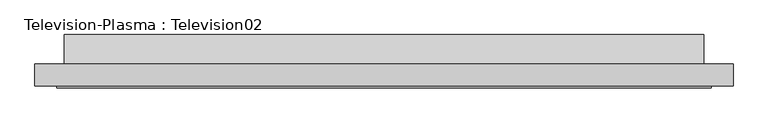
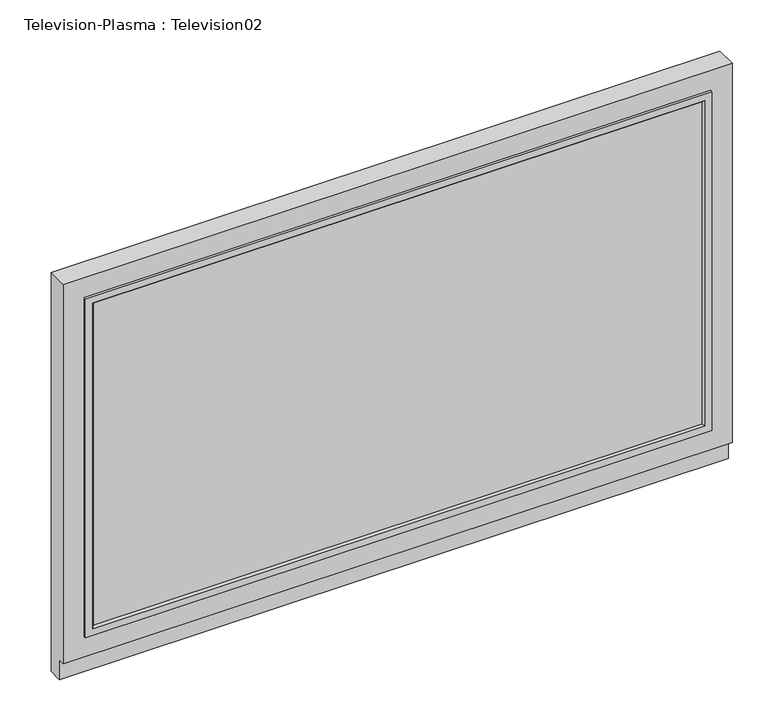
"""IFC4 building model written with IfcOpenShell, lengths in millimetres: furniture geometry, Television-Plasma : Television02."""

import ifcopenshell
import ifcopenshell.guid

model = None  # the IFC model being written
_history = None  # IfcOwnerHistory: only IFC2X3 demands one
_inside = {}  # id of a spatial element -> (the spatial element, [elements in it])
_under = {}  # id of a project, library or spatial element -> (it, [spatial elements below it])
_declared = {}  # id of a project -> (the project, [libraries it declares])
_typed = {}  # id of a type object -> (the type object, [elements of that type])
_made_of = {}  # id of a material, layer set ... -> (it, [elements and type objects made of it])


def new_model(schema):
    """Start an empty IFC model of exactly this schema.

    Asked for "IFC4X3", IfcOpenShell would pick the latest addendum, in which some entities
    have other attributes; the version numbers below select the first issue.
    IFC2X3 requires an IfcOwnerHistory on every rooted entity: one is made here for all.
    """
    global model, _history
    if schema == "IFC4X3":
        model = ifcopenshell.file(schema_version=(4, 3, 0, 0))
    else:
        model = ifcopenshell.file(schema=schema)
    _inside.clear()
    _under.clear()
    _declared.clear()
    _typed.clear()
    _made_of.clear()
    _history = None
    if model.schema == "IFC2X3":
        org = make("IfcOrganization", Name="unknown")
        user = make(
            "IfcPersonAndOrganization",
            ThePerson=make("IfcPerson", FamilyName="unknown"),
            TheOrganization=org,
        )
        app = make(
            "IfcApplication",
            ApplicationDeveloper=org,
            Version="unknown",
            ApplicationFullName="unknown",
            ApplicationIdentifier="unknown",
        )
        _history = make(
            "IfcOwnerHistory",
            OwningUser=user,
            OwningApplication=app,
            ChangeAction="ADDED",
            CreationDate=0,
        )
    return model


def make(cls, **values):
    """One entity of the class cls with the attributes given. An attribute that is None is left unset."""
    return model.create_entity(
        cls, **{name: value for name, value in values.items() if value is not None}
    )


def rooted(cls, **values):
    """An entity with a GlobalId (a new one), such as an element, a storey or a relation."""
    return make(cls, GlobalId=ifcopenshell.guid.new(), OwnerHistory=_history, **values)


def si_unit(unit_type, name, prefix=None):
    """IfcSIUnit, for example si_unit("LENGTHUNIT", "METRE", prefix="MILLI")."""
    return make("IfcSIUnit", UnitType=unit_type, Prefix=prefix, Name=name)


def assignment(units):
    """IfcUnitAssignment: the units of a project."""
    return None if units is None else make("IfcUnitAssignment", Units=units)


def point(xyz):
    """IfcCartesianPoint."""
    return None if xyz is None else make("IfcCartesianPoint", Coordinates=xyz)


def direction(xyz):
    """IfcDirection."""
    return None if xyz is None else make("IfcDirection", DirectionRatios=xyz)


def frame(location, z_axis=None, x_axis=None):
    """IfcAxis2Placement3D, a coordinate frame: its origin and axes. An axis left out is left unset."""
    return make(
        "IfcAxis2Placement3D",
        Location=point(location),
        Axis=direction(z_axis),
        RefDirection=direction(x_axis),
    )


def origin():
    """The frame at (0, 0, 0) with its axes left unset."""
    return frame((0.0, 0.0, 0.0))


def place(relative_to, where):
    """IfcLocalPlacement: puts the frame where relative to a parent placement (None: the world)."""
    return make(
        "IfcLocalPlacement", PlacementRelTo=relative_to, RelativePlacement=where
    )


def context(
    kind, dimensions, precision=None, world=None, true_north=None, identifier=None
):
    """IfcGeometricRepresentationContext, for example the 3D "Model" context."""
    return make(
        "IfcGeometricRepresentationContext",
        ContextIdentifier=identifier,
        ContextType=kind,
        CoordinateSpaceDimension=dimensions,
        Precision=precision,
        WorldCoordinateSystem=world,
        TrueNorth=true_north,
    )


def project(units=None, contexts=None):
    """IfcProject with its units and contexts."""
    return rooted(
        "IfcProject",
        Name="project",
        RepresentationContexts=contexts,
        UnitsInContext=assignment(units),
    )


def spatial(cls, under=None, at=None, **own):
    """A site, building, storey or space (cls), placed at a placement, below another one or the project."""
    s = rooted(cls, ObjectPlacement=at, **own)
    if under is not None:
        _under.setdefault(under.id(), (under, []))[1].append(s)
    return s


def polyline(points):
    """IfcPolyline through the points."""
    return make("IfcPolyline", Points=[point(p) for p in points])


def outline(outer, holes=None, kind="AREA"):
    """IfcArbitraryClosedProfileDef: a profile drawn as a closed curve; with holes, ...WithVoids."""
    if holes is None:
        return make("IfcArbitraryClosedProfileDef", ProfileType=kind, OuterCurve=outer)
    return make(
        "IfcArbitraryProfileDefWithVoids",
        ProfileType=kind,
        OuterCurve=outer,
        InnerCurves=holes,
    )


def extrude(swept, where, along, depth):
    """IfcExtrudedAreaSolid: the profile swept, set in the frame where, extruded along a direction by depth."""
    return make(
        "IfcExtrudedAreaSolid",
        SweptArea=swept,
        Position=where,
        ExtrudedDirection=direction(along),
        Depth=depth,
    )


def faces_of(points, faces, orient=None, outer=None):
    """IfcFace entities. A face is a list of loops; a loop is a list of indices into points, from 0.

    orient and outer hold one flag for each loop. By default every Orientation is true, the
    first loop of a face is its IfcFaceOuterBound and the others are IfcFaceBound.
    """
    made = []
    for i, loops in enumerate(faces):
        bounds = []
        for j, loop in enumerate(loops):
            is_outer = j == 0 if outer is None else outer[i][j]
            bounds.append(
                make(
                    "IfcFaceOuterBound" if is_outer else "IfcFaceBound",
                    Bound=make("IfcPolyLoop", Polygon=[points[k] for k in loop]),
                    Orientation=True if orient is None else orient[i][j],
                )
            )
        made.append(make("IfcFace", Bounds=bounds))
    return made


def faceted_brep(points, faces, orient=None, outer=None, voids=None):
    """IfcFacetedBrep: a solid bounded by flat faces; with voids (closed shells), ...WithVoids."""
    shared = [point(p) for p in points]
    hull = make("IfcClosedShell", CfsFaces=faces_of(shared, faces, orient, outer))
    if voids is None:
        return make("IfcFacetedBrep", Outer=hull)
    return make(
        "IfcFacetedBrepWithVoids",
        Outer=hull,
        Voids=[
            make(cls, CfsFaces=faces_of(shared, fs, o, b)) for cls, fs, o, b in voids
        ],
    )


def shape(context_of_items, identifier, shape_type, items):
    """IfcShapeRepresentation: the items that make up one representation, for example the "Body"."""
    return make(
        "IfcShapeRepresentation",
        ContextOfItems=context_of_items,
        RepresentationIdentifier=identifier,
        RepresentationType=shape_type,
        Items=items,
    )


def source(mapping_origin, context_of_items, identifier, shape_type, items):
    """IfcRepresentationMap: a shape defined once, which mapped items show again and again."""
    return make(
        "IfcRepresentationMap",
        MappingOrigin=mapping_origin,
        MappedRepresentation=shape(context_of_items, identifier, shape_type, items),
    )


def transform(
    local_origin,
    x_axis=None,
    y_axis=None,
    z_axis=None,
    scale=None,
    scale2=None,
    scale3=None,
    uniform=True,
):
    """IfcCartesianTransformationOperator3D, or its non-uniform kind. x_axis, y_axis, z_axis: its Axis1, 2, 3."""
    if uniform:
        return make(
            "IfcCartesianTransformationOperator3D",
            Axis1=direction(x_axis),
            Axis2=direction(y_axis),
            LocalOrigin=point(local_origin),
            Scale=scale,
            Axis3=direction(z_axis),
        )
    return make(
        "IfcCartesianTransformationOperator3DnonUniform",
        Axis1=direction(x_axis),
        Axis2=direction(y_axis),
        LocalOrigin=point(local_origin),
        Scale=scale,
        Axis3=direction(z_axis),
        Scale2=scale2,
        Scale3=scale3,
    )


def mapped(mapping_source, mapping_target):
    """IfcMappedItem: shows the shape of a source again, moved by a transform."""
    return make(
        "IfcMappedItem", MappingSource=mapping_source, MappingTarget=mapping_target
    )


def made_of(thing, what):
    """Note that an element or type object is made of a material, layer set ...; save() writes the relation."""
    if what is not None:
        _made_of.setdefault(what.id(), (what, []))[1].append(thing)
    return thing


def element(
    cls,
    number,
    at=None,
    inside=None,
    cuts=None,
    type_object=None,
    material=None,
    context=None,
    identifier="Body",
    shape_type=None,
    held_by="IfcProductDefinitionShape",
    body=None,
    shapes=None,
    **own,
):
    """One element of the class cls, such as IfcWall. Its Tag is "e" and its number.

    at: its placement. inside: the storey or other place that contains it. cuts: it is an
    opening in that element (IfcRelVoidsElement). A single representation is given by context,
    identifier, shape_type and body (its items); several are given by shapes. held_by: the class
    of the entity that holds the representations. save() writes the other relations.
    """
    e = rooted(cls, Tag="e%d" % number, ObjectPlacement=at, **own)
    if body is not None:
        shapes = [shape(context, identifier, shape_type, body)]
    if shapes is not None:
        e.Representation = make(held_by, Representations=shapes)
    if inside is not None:
        _inside.setdefault(inside.id(), (inside, []))[1].append(e)
    if cuts is not None:
        rooted(
            "IfcRelVoidsElement", RelatingBuildingElement=cuts, RelatedOpeningElement=e
        )
    if type_object is not None:
        _typed.setdefault(type_object.id(), (type_object, []))[1].append(e)
    return made_of(e, material)


def aggregate(whole, parts):
    """IfcRelAggregates: a whole, such as a stair, and the parts it consists of."""
    return rooted("IfcRelAggregates", RelatingObject=whole, RelatedObjects=parts)


def save(model, path):
    """Write the relations noted so far, then the file.

    IfcRelAggregates (storeys below a building ...), IfcRelContainedInSpatialStructure (elements
    in a storey), IfcRelDefinesByType, IfcRelAssociatesMaterial and IfcRelDeclares: one each for
    every whole, place, type object, material and project.
    """
    for whole, parts in _under.values():
        aggregate(whole, parts)
    for where, things in _inside.values():
        rooted(
            "IfcRelContainedInSpatialStructure",
            RelatedElements=things,
            RelatingStructure=where,
        )
    for kind, things in _typed.values():
        rooted("IfcRelDefinesByType", RelatedObjects=things, RelatingType=kind)
    for what, things in _made_of.values():
        rooted("IfcRelAssociatesMaterial", RelatedObjects=things, RelatingMaterial=what)
    for by, libraries in _declared.values():
        rooted("IfcRelDeclares", RelatingContext=by, RelatedDefinitions=libraries)
    model.write(path)


def television_plasma_television02_5b8f3f57(model_context):
    return source(origin(), model_context, "Body", "SolidModel", [
        faceted_brep([(660.4, -50.8, 762.0), (-546.1, -50.8, 762.0), (-546.1, -88.9, 762.0), (660.4, -88.9, 762.0), (-546.1, -50.8, 0.0), (660.4, -50.8, 0.0), (660.4, -76.2, 0.0), (-546.1, -76.2, 0.0), (-495.3, -50.8, 711.2), (-495.3, -50.8, 38.1), (609.6, -50.8, 38.1), (609.6, -50.8, 711.2), (-546.1, -76.2, 38.1), (-546.1, -88.9, 38.1), (660.4, -88.9, 38.1), (-508.0, -88.9, 723.9), (622.3, -88.9, 723.9), (622.3, -88.9, 723.10625), (622.3, -88.9, 76.2), (-508.0, -88.9, 76.2), (-508.0, -88.9, 723.10625), (660.4, -76.2, 38.1), (622.3, -74.1720413, 723.9), (-508.0, -74.1720413, 723.9), (-508.0, -74.1720413, 723.10625), (622.3, -74.1720413, 723.10625), (609.6, -74.1720413, 88.9), (609.6, -74.1720413, 710.40625), (-495.3, -74.1720413, 710.40625), (-495.3, -74.1720413, 88.9), (-495.3, 0.0, 676.4688953), (-495.3, 0.0, 38.1), (609.6, 0.0, 676.4688953), (609.6, 0.0, 38.1), (606.425, -88.9, 92.075), (609.6, -92.075, 88.9), (609.6, -92.075, 710.40625), (606.425, -88.9, 707.23125), (609.6, -88.9, 88.9), (609.6, -88.9, 710.40625), (622.3, -92.075, 723.10625), (622.3, -92.075, 76.2), (-495.3, -92.075, 710.40625), (-492.125, -88.9, 707.23125), (-495.3, -88.9, 710.40625), (-508.0, -92.075, 723.10625), (-495.3, -92.075, 88.9), (-492.125, -88.9, 92.075), (-495.3, -88.9, 88.9), (-508.0, -92.075, 76.2)], [[[0, 1, 2, 3]], [[4, 5, 6, 7]], [[1, 0, 5, 4], [8, 9, 10, 11]], [[2, 1, 4, 7, 12, 13]], [[3, 2, 13, 14], [15, 16, 17, 18, 19, 20]], [[0, 3, 14, 21, 6, 5]], [[22, 23, 24, 25]], [[26, 27, 28, 29]], [[16, 22, 25, 17]], [[23, 15, 20, 24]], [[23, 22, 16, 15]], [[21, 12, 7, 6]], [[12, 21, 14, 13]], [[30, 31, 9, 8]], [[32, 11, 10, 33]], [[31, 30, 32, 33]], [[9, 31, 33, 10]], [[30, 8, 11, 32]], [[34, 35, 36, 37]], [[26, 38, 39, 27]], [[40, 41, 18, 17]], [[37, 36, 42, 43]], [[27, 39, 44, 28]], [[45, 40, 17, 25, 24, 20]], [[43, 42, 46, 47]], [[28, 44, 48, 29]], [[49, 45, 20, 19]], [[41, 40, 45, 49], [36, 35, 46, 42]], [[35, 34, 47, 46]], [[39, 38, 48, 44], [34, 37, 43, 47]], [[38, 26, 29, 48]], [[41, 49, 19, 18]]]),
        extrude(outline(polyline([(609.6, -88.9), (-495.3, -88.9), (-495.3, -74.1720413), (609.6, -74.1720413), (609.6, -88.9)])), frame((0.0, 0.0, 88.9), z_axis=(0.0, 0.0, 1.0), x_axis=(1.0, 0.0, 0.0)), (0.0, 0.0, 1.0), 622.3),
    ])


if __name__ == "__main__":
    model = new_model("IFC4")
    model_context = context("Model", 3, world=origin())
    ifc_project = project(units=[si_unit("LENGTHUNIT", "METRE", prefix="MILLI")], contexts=[model_context])
    site = spatial("IfcSite", under=ifc_project)
    building = spatial("IfcBuilding", under=site)
    placement = place(None, origin())
    television_plasma_television02_shape = television_plasma_television02_5b8f3f57(model_context)
    element("IfcFurniture", 1, ObjectType="Television-Plasma : Television02", at=placement, inside=building, context=model_context, shape_type="MappedRepresentation", body=[
        mapped(television_plasma_television02_shape, transform((0.0, 0.0, 0.0), x_axis=(1.0, 0.0, 0.0), y_axis=(0.0, 1.0, 0.0), z_axis=(0.0, 0.0, 1.0))),
    ])
    save(model, "model.ifc")

# Revit data of these elements
# Type "Television-Plasma : Television02"
#   Assembly Code = "E2020200"
#   Width = 3' - 11 1/2"
#   Height = 2' - 6"
#   Depth = 0' - 3 1/2"
#   Cabinet Material = Plastic - Gray
#   Default Elevation = 0
# Element 1 (IfcFurniture, "Television-Plasma : Television02")
#   Materials on its faces: "Plastic - Gray", "Glass"
# Materials
#   "Plastic - Gray": class "Unassigned", colour RGB 134 134 134, transparency 0
#   "Glass": class "Unassigned", colour RGB 0 128 192, transparency 0.75
